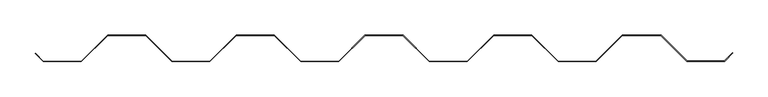
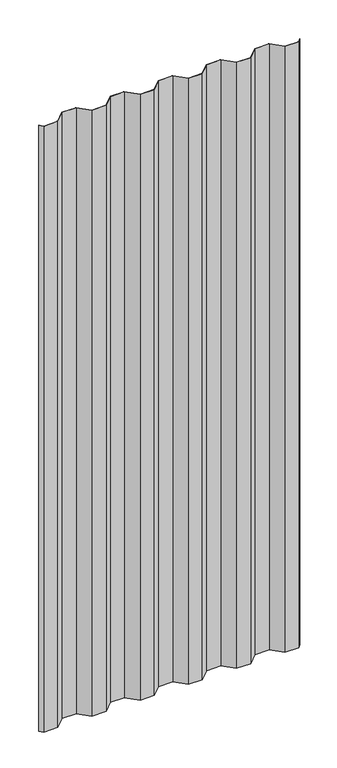
"""IFC4 building model written with IfcOpenShell, lengths in millimetres: proxy geometry, MBCI 7.2-V Panel2 : MBCI 7.2-V Panel-1."""

import ifcopenshell
import ifcopenshell.guid

model = None  # the IFC model being written
_history = None  # IfcOwnerHistory: only IFC2X3 demands one
_inside = {}  # id of a spatial element -> (the spatial element, [elements in it])
_under = {}  # id of a project, library or spatial element -> (it, [spatial elements below it])
_declared = {}  # id of a project -> (the project, [libraries it declares])
_typed = {}  # id of a type object -> (the type object, [elements of that type])
_made_of = {}  # id of a material, layer set ... -> (it, [elements and type objects made of it])


def new_model(schema):
    """Start an empty IFC model of exactly this schema.

    Asked for "IFC4X3", IfcOpenShell would pick the latest addendum, in which some entities
    have other attributes; the version numbers below select the first issue.
    IFC2X3 requires an IfcOwnerHistory on every rooted entity: one is made here for all.
    """
    global model, _history
    if schema == "IFC4X3":
        model = ifcopenshell.file(schema_version=(4, 3, 0, 0))
    else:
        model = ifcopenshell.file(schema=schema)
    _inside.clear()
    _under.clear()
    _declared.clear()
    _typed.clear()
    _made_of.clear()
    _history = None
    if model.schema == "IFC2X3":
        org = make("IfcOrganization", Name="unknown")
        user = make(
            "IfcPersonAndOrganization",
            ThePerson=make("IfcPerson", FamilyName="unknown"),
            TheOrganization=org,
        )
        app = make(
            "IfcApplication",
            ApplicationDeveloper=org,
            Version="unknown",
            ApplicationFullName="unknown",
            ApplicationIdentifier="unknown",
        )
        _history = make(
            "IfcOwnerHistory",
            OwningUser=user,
            OwningApplication=app,
            ChangeAction="ADDED",
            CreationDate=0,
        )
    return model


def make(cls, **values):
    """One entity of the class cls with the attributes given. An attribute that is None is left unset."""
    return model.create_entity(
        cls, **{name: value for name, value in values.items() if value is not None}
    )


def rooted(cls, **values):
    """An entity with a GlobalId (a new one), such as an element, a storey or a relation."""
    return make(cls, GlobalId=ifcopenshell.guid.new(), OwnerHistory=_history, **values)


def si_unit(unit_type, name, prefix=None):
    """IfcSIUnit, for example si_unit("LENGTHUNIT", "METRE", prefix="MILLI")."""
    return make("IfcSIUnit", UnitType=unit_type, Prefix=prefix, Name=name)


def assignment(units):
    """IfcUnitAssignment: the units of a project."""
    return None if units is None else make("IfcUnitAssignment", Units=units)


def point(xyz):
    """IfcCartesianPoint."""
    return None if xyz is None else make("IfcCartesianPoint", Coordinates=xyz)


def direction(xyz):
    """IfcDirection."""
    return None if xyz is None else make("IfcDirection", DirectionRatios=xyz)


def frame(location, z_axis=None, x_axis=None):
    """IfcAxis2Placement3D, a coordinate frame: its origin and axes. An axis left out is left unset."""
    return make(
        "IfcAxis2Placement3D",
        Location=point(location),
        Axis=direction(z_axis),
        RefDirection=direction(x_axis),
    )


def origin():
    """The frame at (0, 0, 0) with its axes left unset."""
    return frame((0.0, 0.0, 0.0))


def place(relative_to, where):
    """IfcLocalPlacement: puts the frame where relative to a parent placement (None: the world)."""
    return make(
        "IfcLocalPlacement", PlacementRelTo=relative_to, RelativePlacement=where
    )


def context(
    kind, dimensions, precision=None, world=None, true_north=None, identifier=None
):
    """IfcGeometricRepresentationContext, for example the 3D "Model" context."""
    return make(
        "IfcGeometricRepresentationContext",
        ContextIdentifier=identifier,
        ContextType=kind,
        CoordinateSpaceDimension=dimensions,
        Precision=precision,
        WorldCoordinateSystem=world,
        TrueNorth=true_north,
    )


def project(units=None, contexts=None):
    """IfcProject with its units and contexts."""
    return rooted(
        "IfcProject",
        Name="project",
        RepresentationContexts=contexts,
        UnitsInContext=assignment(units),
    )


def spatial(cls, under=None, at=None, **own):
    """A site, building, storey or space (cls), placed at a placement, below another one or the project."""
    s = rooted(cls, ObjectPlacement=at, **own)
    if under is not None:
        _under.setdefault(under.id(), (under, []))[1].append(s)
    return s


def polyline(points):
    """IfcPolyline through the points."""
    return make("IfcPolyline", Points=[point(p) for p in points])


def outline(outer, holes=None, kind="AREA"):
    """IfcArbitraryClosedProfileDef: a profile drawn as a closed curve; with holes, ...WithVoids."""
    if holes is None:
        return make("IfcArbitraryClosedProfileDef", ProfileType=kind, OuterCurve=outer)
    return make(
        "IfcArbitraryProfileDefWithVoids",
        ProfileType=kind,
        OuterCurve=outer,
        InnerCurves=holes,
    )


def extrude(swept, where, along, depth):
    """IfcExtrudedAreaSolid: the profile swept, set in the frame where, extruded along a direction by depth."""
    return make(
        "IfcExtrudedAreaSolid",
        SweptArea=swept,
        Position=where,
        ExtrudedDirection=direction(along),
        Depth=depth,
    )


def shape(context_of_items, identifier, shape_type, items):
    """IfcShapeRepresentation: the items that make up one representation, for example the "Body"."""
    return make(
        "IfcShapeRepresentation",
        ContextOfItems=context_of_items,
        RepresentationIdentifier=identifier,
        RepresentationType=shape_type,
        Items=items,
    )


def source(mapping_origin, context_of_items, identifier, shape_type, items):
    """IfcRepresentationMap: a shape defined once, which mapped items show again and again."""
    return make(
        "IfcRepresentationMap",
        MappingOrigin=mapping_origin,
        MappedRepresentation=shape(context_of_items, identifier, shape_type, items),
    )


def transform(
    local_origin,
    x_axis=None,
    y_axis=None,
    z_axis=None,
    scale=None,
    scale2=None,
    scale3=None,
    uniform=True,
):
    """IfcCartesianTransformationOperator3D, or its non-uniform kind. x_axis, y_axis, z_axis: its Axis1, 2, 3."""
    if uniform:
        return make(
            "IfcCartesianTransformationOperator3D",
            Axis1=direction(x_axis),
            Axis2=direction(y_axis),
            LocalOrigin=point(local_origin),
            Scale=scale,
            Axis3=direction(z_axis),
        )
    return make(
        "IfcCartesianTransformationOperator3DnonUniform",
        Axis1=direction(x_axis),
        Axis2=direction(y_axis),
        LocalOrigin=point(local_origin),
        Scale=scale,
        Axis3=direction(z_axis),
        Scale2=scale2,
        Scale3=scale3,
    )


def mapped(mapping_source, mapping_target):
    """IfcMappedItem: shows the shape of a source again, moved by a transform."""
    return make(
        "IfcMappedItem", MappingSource=mapping_source, MappingTarget=mapping_target
    )


def made_of(thing, what):
    """Note that an element or type object is made of a material, layer set ...; save() writes the relation."""
    if what is not None:
        _made_of.setdefault(what.id(), (what, []))[1].append(thing)
    return thing


def element(
    cls,
    number,
    at=None,
    inside=None,
    cuts=None,
    type_object=None,
    material=None,
    context=None,
    identifier="Body",
    shape_type=None,
    held_by="IfcProductDefinitionShape",
    body=None,
    shapes=None,
    **own,
):
    """One element of the class cls, such as IfcWall. Its Tag is "e" and its number.

    at: its placement. inside: the storey or other place that contains it. cuts: it is an
    opening in that element (IfcRelVoidsElement). A single representation is given by context,
    identifier, shape_type and body (its items); several are given by shapes. held_by: the class
    of the entity that holds the representations. save() writes the other relations.
    """
    e = rooted(cls, Tag="e%d" % number, ObjectPlacement=at, **own)
    if body is not None:
        shapes = [shape(context, identifier, shape_type, body)]
    if shapes is not None:
        e.Representation = make(held_by, Representations=shapes)
    if inside is not None:
        _inside.setdefault(inside.id(), (inside, []))[1].append(e)
    if cuts is not None:
        rooted(
            "IfcRelVoidsElement", RelatingBuildingElement=cuts, RelatedOpeningElement=e
        )
    if type_object is not None:
        _typed.setdefault(type_object.id(), (type_object, []))[1].append(e)
    return made_of(e, material)


def aggregate(whole, parts):
    """IfcRelAggregates: a whole, such as a stair, and the parts it consists of."""
    return rooted("IfcRelAggregates", RelatingObject=whole, RelatedObjects=parts)


def save(model, path):
    """Write the relations noted so far, then the file.

    IfcRelAggregates (storeys below a building ...), IfcRelContainedInSpatialStructure (elements
    in a storey), IfcRelDefinesByType, IfcRelAssociatesMaterial and IfcRelDeclares: one each for
    every whole, place, type object, material and project.
    """
    for whole, parts in _under.values():
        aggregate(whole, parts)
    for where, things in _inside.values():
        rooted(
            "IfcRelContainedInSpatialStructure",
            RelatedElements=things,
            RelatingStructure=where,
        )
    for kind, things in _typed.values():
        rooted("IfcRelDefinesByType", RelatedObjects=things, RelatingType=kind)
    for what, things in _made_of.values():
        rooted("IfcRelAssociatesMaterial", RelatedObjects=things, RelatingMaterial=what)
    for by, libraries in _declared.values():
        rooted("IfcRelDeclares", RelatingContext=by, RelatedDefinitions=libraries)
    model.write(path)


def generic_models_5825bab2(model_context):
    return source(origin(), model_context, "Body", "SweptSolid", [
        extrude(outline(polyline([(588241.1303729, -531639.2163841), (588187.0186638, -531639.2163841), (588175.6180296, -531627.81575), (588176.4180038, -531627.7738251), (588187.2652503, -531638.6210716), (588240.8837864, -531638.6210716), (588278.3741864, -531601.1306716), (588332.6548503, -531601.1306716), (588370.1452503, -531638.6210716), (588423.7637864, -531638.6210716), (588461.2541864, -531601.1306716), (588515.5348503, -531601.1306716), (588553.0252503, -531638.6210716), (588606.6437864, -531638.6210716), (588644.1341864, -531601.1306716), (588698.4148503, -531601.1306716), (588735.9052503, -531638.6210716), (588789.5237864, -531638.6210716), (588827.0141864, -531601.1306716), (588881.2948503, -531601.1306716), (588918.7852503, -531638.6210716), (588972.4037864, -531638.6210716), (589009.8941864, -531601.1306716), (589065.0384503, -531601.1306716), (589101.9192503, -531638.0114716), (589155.0073773, -531638.0114716), (589166.1378112, -531626.8810377), (589166.9246865, -531626.9360614), (589155.2539638, -531638.6067841), (589101.6726638, -531638.6067841), (589064.7918638, -531601.7259841), (589010.1407729, -531601.7259841), (588972.6503729, -531639.2163841), (588918.5386638, -531639.2163841), (588881.0482638, -531601.7259841), (588827.2607729, -531601.7259841), (588789.7703729, -531639.2163841), (588735.6586638, -531639.2163841), (588698.1682638, -531601.7259841), (588644.3807729, -531601.7259841), (588606.8903729, -531639.2163841), (588552.7786638, -531639.2163841), (588515.2882638, -531601.7259841), (588461.5007729, -531601.7259841), (588424.0103729, -531639.2163841), (588369.8986638, -531639.2163841), (588332.4082638, -531601.7259841), (588278.6207729, -531601.7259841), (588241.1303729, -531639.2163841)])), frame((0.0, 0.0, 6.35), z_axis=(0.0, 0.0, 1.0), x_axis=(1.0, 0.0, 0.0)), (0.0, 0.0, 1.0), 2432.05),
    ])


if __name__ == "__main__":
    model = new_model("IFC4")
    model_context = context("Model", 3, world=origin())
    ifc_project = project(units=[si_unit("LENGTHUNIT", "METRE", prefix="MILLI")], contexts=[model_context])
    site = spatial("IfcSite", under=ifc_project)
    building = spatial("IfcBuilding", under=site)
    placement = place(None, origin())
    generic_models_shape = generic_models_5825bab2(model_context)
    element("IfcBuildingElementProxy", 1, Name="MBCI 7.2-V Panel2 : MBCI 7.2-V Panel-1", ObjectType="MBCI 7.2-V Panel2 : MBCI 7.2-V Panel-1", at=placement, inside=building, context=model_context, shape_type="MappedRepresentation", body=[
        mapped(generic_models_shape, transform((0.0, 0.0, 0.0), x_axis=(1.0, 0.0, 0.0), y_axis=(0.0, 1.0, 0.0), z_axis=(0.0, 0.0, 1.0))),
    ])
    save(model, "model.ifc")

# Revit data of these elements
# Element 1 (IfcBuildingElementProxy, "MBCI 7.2-V Panel2 : MBCI 7.2-V Panel-1")
#   Materials on its faces: "MTL PANEL"
# Materials
#   "MTL PANEL": class "Generic", colour RGB 239 242 240, transparency 0, Cost = 0
